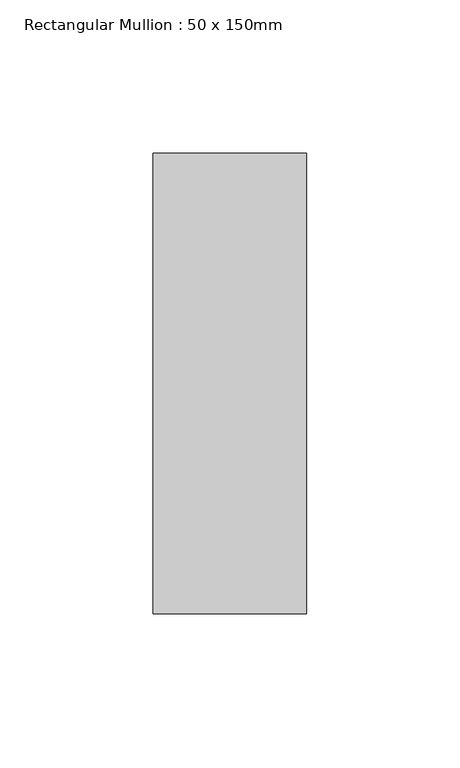
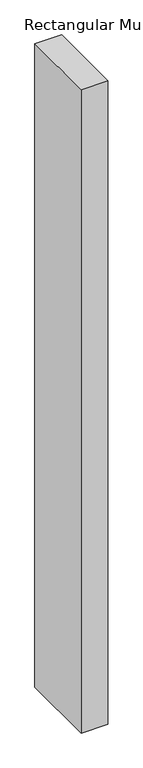
"""IFC4 building model written with IfcOpenShell, lengths in millimetres: member geometry, Rectangular Mullion : 50 x 150mm."""

from ifc_helpers import new_model, si_unit, frame, origin, place, context, project, spatial, polyline, outline, extrude, source, transform, mapped, element, save


def rectangular_mullion_50_x_150mm_345eee08(model_context):
    return source(origin(), model_context, "Body", "SweptSolid", [
        extrude(outline(polyline([(0.0, 75.0), (0.0, -75.0), (-50.0, -75.0), (-50.0, 75.0), (0.0, 75.0)])), frame((0.0, 0.0, -1274.9999998), z_axis=(0.0, 0.0, 1.0), x_axis=(1.0, 0.0, 0.0)), (0.0, 0.0, 1.0), 1274.9999998),
    ])


if __name__ == "__main__":
    model = new_model("IFC4")
    model_context = context("Model", 3, world=origin())
    ifc_project = project(units=[si_unit("LENGTHUNIT", "METRE", prefix="MILLI")], contexts=[model_context])
    site = spatial("IfcSite", under=ifc_project)
    building = spatial("IfcBuilding", under=site)
    placement = place(None, origin())
    rectangular_mullion_50_x_150mm_shape = rectangular_mullion_50_x_150mm_345eee08(model_context)
    element("IfcMember", 1, ObjectType="Rectangular Mullion : 50 x 150mm", at=placement, inside=building, context=model_context, shape_type="MappedRepresentation", body=[
        mapped(rectangular_mullion_50_x_150mm_shape, transform((0.0, 0.0, 0.0), x_axis=(1.0, 0.0, 0.0), y_axis=(0.0, 1.0, 0.0), z_axis=(0.0, 0.0, 1.0))),
    ])
    save(model, "model.ifc")

# Revit data of these elements
# Type "Rectangular Mullion : 50 x 150mm"
#   built-in parameter 1007304 = 0.492126 (stored number, unit not read)
#   built-in parameter 1007301 = 0.082021 (stored number, unit not read)
#   built-in parameter 1007300 = 0.082021 (stored number, unit not read)
# Element 1 (IfcMember, "Rectangular Mullion : 50 x 150mm")
#   Materials on its faces: "Aluminium"
# Materials
#   "Aluminium": class "Metal", colour RGB 247 247 247, transparency 0, Description = "Aluminium 6061", Cost = 0
